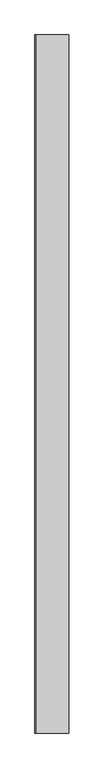
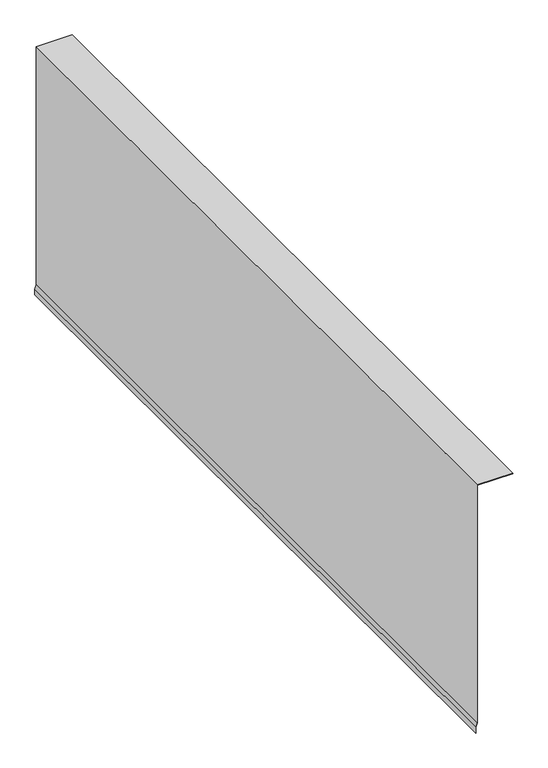
"""IFC4 building model written with IfcOpenShell, lengths in millimetres: proxy geometry, Membrane056 4504 : Membrane056 4504."""

import ifcopenshell
import ifcopenshell.guid

model = None  # the IFC model being written
_history = None  # IfcOwnerHistory: only IFC2X3 demands one
_inside = {}  # id of a spatial element -> (the spatial element, [elements in it])
_under = {}  # id of a project, library or spatial element -> (it, [spatial elements below it])
_declared = {}  # id of a project -> (the project, [libraries it declares])
_typed = {}  # id of a type object -> (the type object, [elements of that type])
_made_of = {}  # id of a material, layer set ... -> (it, [elements and type objects made of it])


def new_model(schema):
    """Start an empty IFC model of exactly this schema.

    Asked for "IFC4X3", IfcOpenShell would pick the latest addendum, in which some entities
    have other attributes; the version numbers below select the first issue.
    IFC2X3 requires an IfcOwnerHistory on every rooted entity: one is made here for all.
    """
    global model, _history
    if schema == "IFC4X3":
        model = ifcopenshell.file(schema_version=(4, 3, 0, 0))
    else:
        model = ifcopenshell.file(schema=schema)
    _inside.clear()
    _under.clear()
    _declared.clear()
    _typed.clear()
    _made_of.clear()
    _history = None
    if model.schema == "IFC2X3":
        org = make("IfcOrganization", Name="unknown")
        user = make(
            "IfcPersonAndOrganization",
            ThePerson=make("IfcPerson", FamilyName="unknown"),
            TheOrganization=org,
        )
        app = make(
            "IfcApplication",
            ApplicationDeveloper=org,
            Version="unknown",
            ApplicationFullName="unknown",
            ApplicationIdentifier="unknown",
        )
        _history = make(
            "IfcOwnerHistory",
            OwningUser=user,
            OwningApplication=app,
            ChangeAction="ADDED",
            CreationDate=0,
        )
    return model


def make(cls, **values):
    """One entity of the class cls with the attributes given. An attribute that is None is left unset."""
    return model.create_entity(
        cls, **{name: value for name, value in values.items() if value is not None}
    )


def rooted(cls, **values):
    """An entity with a GlobalId (a new one), such as an element, a storey or a relation."""
    return make(cls, GlobalId=ifcopenshell.guid.new(), OwnerHistory=_history, **values)


def si_unit(unit_type, name, prefix=None):
    """IfcSIUnit, for example si_unit("LENGTHUNIT", "METRE", prefix="MILLI")."""
    return make("IfcSIUnit", UnitType=unit_type, Prefix=prefix, Name=name)


def assignment(units):
    """IfcUnitAssignment: the units of a project."""
    return None if units is None else make("IfcUnitAssignment", Units=units)


def point(xyz):
    """IfcCartesianPoint."""
    return None if xyz is None else make("IfcCartesianPoint", Coordinates=xyz)


def direction(xyz):
    """IfcDirection."""
    return None if xyz is None else make("IfcDirection", DirectionRatios=xyz)


def frame(location, z_axis=None, x_axis=None):
    """IfcAxis2Placement3D, a coordinate frame: its origin and axes. An axis left out is left unset."""
    return make(
        "IfcAxis2Placement3D",
        Location=point(location),
        Axis=direction(z_axis),
        RefDirection=direction(x_axis),
    )


def origin():
    """The frame at (0, 0, 0) with its axes left unset."""
    return frame((0.0, 0.0, 0.0))


def place(relative_to, where):
    """IfcLocalPlacement: puts the frame where relative to a parent placement (None: the world)."""
    return make(
        "IfcLocalPlacement", PlacementRelTo=relative_to, RelativePlacement=where
    )


def context(
    kind, dimensions, precision=None, world=None, true_north=None, identifier=None
):
    """IfcGeometricRepresentationContext, for example the 3D "Model" context."""
    return make(
        "IfcGeometricRepresentationContext",
        ContextIdentifier=identifier,
        ContextType=kind,
        CoordinateSpaceDimension=dimensions,
        Precision=precision,
        WorldCoordinateSystem=world,
        TrueNorth=true_north,
    )


def project(units=None, contexts=None):
    """IfcProject with its units and contexts."""
    return rooted(
        "IfcProject",
        Name="project",
        RepresentationContexts=contexts,
        UnitsInContext=assignment(units),
    )


def spatial(cls, under=None, at=None, **own):
    """A site, building, storey or space (cls), placed at a placement, below another one or the project."""
    s = rooted(cls, ObjectPlacement=at, **own)
    if under is not None:
        _under.setdefault(under.id(), (under, []))[1].append(s)
    return s


def polyline(points):
    """IfcPolyline through the points."""
    return make("IfcPolyline", Points=[point(p) for p in points])


def outline(outer, holes=None, kind="AREA"):
    """IfcArbitraryClosedProfileDef: a profile drawn as a closed curve; with holes, ...WithVoids."""
    if holes is None:
        return make("IfcArbitraryClosedProfileDef", ProfileType=kind, OuterCurve=outer)
    return make(
        "IfcArbitraryProfileDefWithVoids",
        ProfileType=kind,
        OuterCurve=outer,
        InnerCurves=holes,
    )


def extrude(swept, where, along, depth):
    """IfcExtrudedAreaSolid: the profile swept, set in the frame where, extruded along a direction by depth."""
    return make(
        "IfcExtrudedAreaSolid",
        SweptArea=swept,
        Position=where,
        ExtrudedDirection=direction(along),
        Depth=depth,
    )


def shape(context_of_items, identifier, shape_type, items):
    """IfcShapeRepresentation: the items that make up one representation, for example the "Body"."""
    return make(
        "IfcShapeRepresentation",
        ContextOfItems=context_of_items,
        RepresentationIdentifier=identifier,
        RepresentationType=shape_type,
        Items=items,
    )


def source(mapping_origin, context_of_items, identifier, shape_type, items):
    """IfcRepresentationMap: a shape defined once, which mapped items show again and again."""
    return make(
        "IfcRepresentationMap",
        MappingOrigin=mapping_origin,
        MappedRepresentation=shape(context_of_items, identifier, shape_type, items),
    )


def transform(
    local_origin,
    x_axis=None,
    y_axis=None,
    z_axis=None,
    scale=None,
    scale2=None,
    scale3=None,
    uniform=True,
):
    """IfcCartesianTransformationOperator3D, or its non-uniform kind. x_axis, y_axis, z_axis: its Axis1, 2, 3."""
    if uniform:
        return make(
            "IfcCartesianTransformationOperator3D",
            Axis1=direction(x_axis),
            Axis2=direction(y_axis),
            LocalOrigin=point(local_origin),
            Scale=scale,
            Axis3=direction(z_axis),
        )
    return make(
        "IfcCartesianTransformationOperator3DnonUniform",
        Axis1=direction(x_axis),
        Axis2=direction(y_axis),
        LocalOrigin=point(local_origin),
        Scale=scale,
        Axis3=direction(z_axis),
        Scale2=scale2,
        Scale3=scale3,
    )


def mapped(mapping_source, mapping_target):
    """IfcMappedItem: shows the shape of a source again, moved by a transform."""
    return make(
        "IfcMappedItem", MappingSource=mapping_source, MappingTarget=mapping_target
    )


def made_of(thing, what):
    """Note that an element or type object is made of a material, layer set ...; save() writes the relation."""
    if what is not None:
        _made_of.setdefault(what.id(), (what, []))[1].append(thing)
    return thing


def element(
    cls,
    number,
    at=None,
    inside=None,
    cuts=None,
    type_object=None,
    material=None,
    context=None,
    identifier="Body",
    shape_type=None,
    held_by="IfcProductDefinitionShape",
    body=None,
    shapes=None,
    **own,
):
    """One element of the class cls, such as IfcWall. Its Tag is "e" and its number.

    at: its placement. inside: the storey or other place that contains it. cuts: it is an
    opening in that element (IfcRelVoidsElement). A single representation is given by context,
    identifier, shape_type and body (its items); several are given by shapes. held_by: the class
    of the entity that holds the representations. save() writes the other relations.
    """
    e = rooted(cls, Tag="e%d" % number, ObjectPlacement=at, **own)
    if body is not None:
        shapes = [shape(context, identifier, shape_type, body)]
    if shapes is not None:
        e.Representation = make(held_by, Representations=shapes)
    if inside is not None:
        _inside.setdefault(inside.id(), (inside, []))[1].append(e)
    if cuts is not None:
        rooted(
            "IfcRelVoidsElement", RelatingBuildingElement=cuts, RelatedOpeningElement=e
        )
    if type_object is not None:
        _typed.setdefault(type_object.id(), (type_object, []))[1].append(e)
    return made_of(e, material)


def aggregate(whole, parts):
    """IfcRelAggregates: a whole, such as a stair, and the parts it consists of."""
    return rooted("IfcRelAggregates", RelatingObject=whole, RelatedObjects=parts)


def save(model, path):
    """Write the relations noted so far, then the file.

    IfcRelAggregates (storeys below a building ...), IfcRelContainedInSpatialStructure (elements
    in a storey), IfcRelDefinesByType, IfcRelAssociatesMaterial and IfcRelDeclares: one each for
    every whole, place, type object, material and project.
    """
    for whole, parts in _under.values():
        aggregate(whole, parts)
    for where, things in _inside.values():
        rooted(
            "IfcRelContainedInSpatialStructure",
            RelatedElements=things,
            RelatingStructure=where,
        )
    for kind, things in _typed.values():
        rooted("IfcRelDefinesByType", RelatedObjects=things, RelatingType=kind)
    for what, things in _made_of.values():
        rooted("IfcRelAssociatesMaterial", RelatedObjects=things, RelatingMaterial=what)
    for by, libraries in _declared.values():
        rooted("IfcRelDeclares", RelatingContext=by, RelatedDefinitions=libraries)
    model.write(path)


def generic_models_68b2d0ef(model_context):
    return source(origin(), model_context, "Body", "SweptSolid", [
        extrude(outline(polyline([(40237.828125, -4904.6197981), (40237.828125, -4998.1919031), (39579.4993977, -4998.1919031), (39568.2741325, -5002.2775655), (39552.6918208, -5002.2775655), (39552.6918208, -5001.2775655), (39568.0978055, -5001.2775655), (39579.3230707, -4997.1919031), (40236.828125, -4997.1919031), (40236.828125, -4904.6197981), (40237.828125, -4904.6197981)])), frame((0.0, -1052.8906574, 0.0), z_axis=(0.0, 1.0, 0.0), x_axis=(0.0, 0.0, 1.0)), (0.0, 0.0, 1.0), 2000.0),
    ])


if __name__ == "__main__":
    model = new_model("IFC4")
    model_context = context("Model", 3, world=origin())
    ifc_project = project(units=[si_unit("LENGTHUNIT", "METRE", prefix="MILLI")], contexts=[model_context])
    site = spatial("IfcSite", under=ifc_project)
    building = spatial("IfcBuilding", under=site)
    placement = place(None, origin())
    generic_models_shape = generic_models_68b2d0ef(model_context)
    element("IfcBuildingElementProxy", 1, Name="Membrane056 4504 : Membrane056 4504", ObjectType="Membrane056 4504 : Membrane056 4504", at=placement, inside=building, context=model_context, shape_type="MappedRepresentation", body=[
        mapped(generic_models_shape, transform((0.0, 0.0, 0.0), x_axis=(1.0, 0.0, 0.0), y_axis=(0.0, 1.0, 0.0), z_axis=(0.0, 0.0, 1.0))),
    ])
    save(model, "model.ifc")

# Revit data of these elements
# Type "Membrane056 4504 : Membrane056 4504"
#   NameOverride = "Membrane056"
# Element 1 (IfcBuildingElementProxy, "Membrane056 4504 : Membrane056 4504")
#   Materials on its faces: "2 LAYERS NO. 30 ASTM D226 ASPHALT SATURATED ORGANIC FELT"
# Materials
#   "2 LAYERS NO. 30 ASTM D226 ASPHALT SATURATED ORGANIC FELT": class "Unassigned", colour RGB 46 171 0, transparency 0
